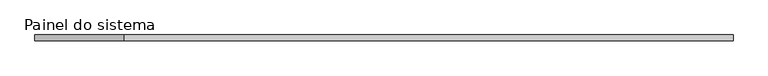
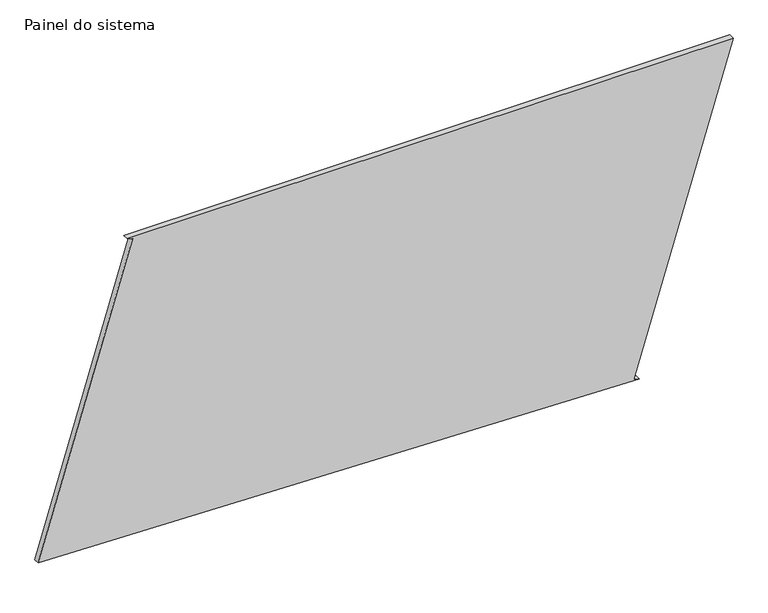
"""IFC4 building model written with IfcOpenShell, lengths in millimetres: plate geometry, Painel do sistema : Envidraçado."""

from ifc_helpers import new_model, si_unit, frame, origin, place, context, project, spatial, polyline, outline, extrude, source, transform, mapped, element, save


def painel_do_sistema_5fa93e6e(model_context):
    return source(origin(), model_context, "Body", "SweptSolid", [
        extrude(outline(polyline([(0.0, 1114.6784136), (7.2712141, 1090.7591861), (1441.1773173, 1526.6527883), (1441.1773173, -1136.0888645), (1433.9061032, -1112.1696369), (70.4313529, -1526.6527883), (0.0, 1114.6784136)])), frame((0.0, 24.5, 0.0), z_axis=(0.0, 1.0, 0.0), x_axis=(0.0, 0.0, 1.0)), (0.0, 0.0, 1.0), 25.0),
    ])


if __name__ == "__main__":
    model = new_model("IFC4")
    model_context = context("Model", 3, world=origin())
    ifc_project = project(units=[si_unit("LENGTHUNIT", "METRE", prefix="MILLI")], contexts=[model_context])
    site = spatial("IfcSite", under=ifc_project)
    building = spatial("IfcBuilding", under=site)
    placement = place(None, origin())
    painel_do_sistema_shape = painel_do_sistema_5fa93e6e(model_context)
    element("IfcPlate", 1, ObjectType="Painel do sistema : Envidraçado", at=placement, inside=building, context=model_context, shape_type="MappedRepresentation", body=[
        mapped(painel_do_sistema_shape, transform((0.0, 0.0, 0.0), x_axis=(1.0, 0.0, 0.0), y_axis=(0.0, 1.0, 0.0), z_axis=(0.0, 0.0, 1.0))),
    ])
    save(model, "model.ifc")

# Revit data of these elements
# Type "Painel do sistema : Envidraçado"
#   Construction Type Id = "GSP4R"
#   Analytic Construction = "Vidraça única Pilkington 1/8 pol"
#   Visual Light Transmittance = 0.9
#   Solar Heat Gain Coefficient = 0.86
#   Heat Transfer Coefficient (U) = 6.7069 W/(m²·K)
# Element 1 (IfcPlate, "Painel do sistema : Envidraçado")
#   Materials on its faces: "Vidro"
# Materials
#   "Vidro": class "Vidro", colour RGB 0 128 192, transparency 0.9, Description = "Vidro de sílica", Cost = 0
